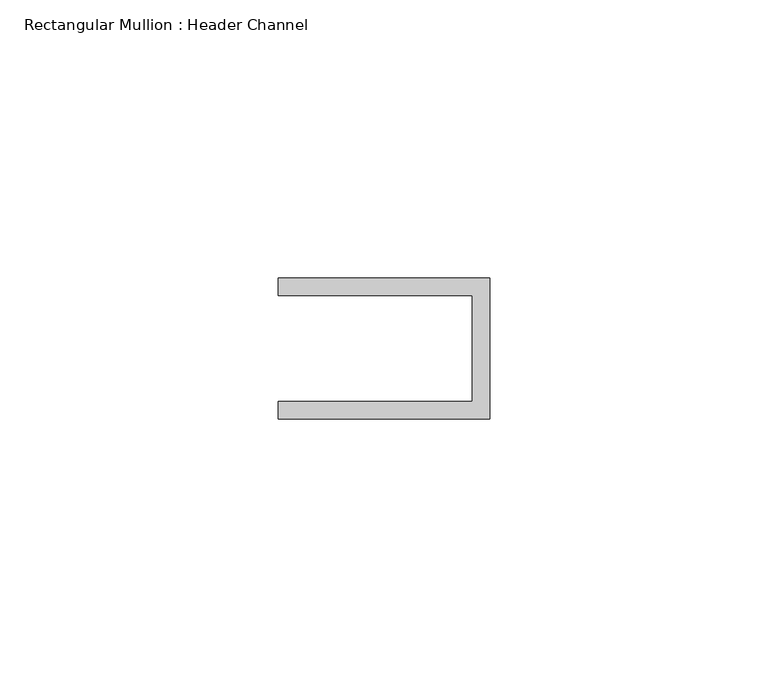
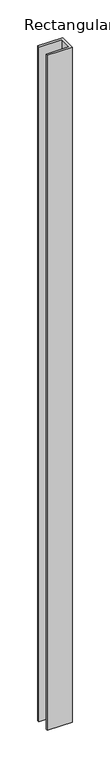
"""IFC4 building model written with IfcOpenShell, lengths in millimetres: member geometry, Rectangular Mullion : Header Channel."""

from ifc_helpers import new_model, si_unit, frame, origin, place, context, project, spatial, polyline, outline, extrude, source, transform, mapped, element, save


def rectangular_mullion_header_channel_626751b6(model_context):
    return source(origin(), model_context, "Body", "SweptSolid", [
        extrude(outline(polyline([(0.0, -12.7), (-38.1, -12.7), (-38.1, -9.525), (-3.175, -9.525), (-3.175, 9.525), (-38.1, 9.525), (-38.1, 12.7), (0.0, 12.7), (0.0, -12.7)])), frame((0.0, 0.0, -1092.2), z_axis=(0.0, 0.0, 1.0), x_axis=(1.0, 0.0, 0.0)), (0.0, 0.0, 1.0), 1092.2),
    ])


if __name__ == "__main__":
    model = new_model("IFC4")
    model_context = context("Model", 3, world=origin())
    ifc_project = project(units=[si_unit("LENGTHUNIT", "METRE", prefix="MILLI")], contexts=[model_context])
    site = spatial("IfcSite", under=ifc_project)
    building = spatial("IfcBuilding", under=site)
    placement = place(None, origin())
    rectangular_mullion_header_channel_shape = rectangular_mullion_header_channel_626751b6(model_context)
    element("IfcMember", 1, ObjectType="Rectangular Mullion : Header Channel", at=placement, inside=building, context=model_context, shape_type="MappedRepresentation", body=[
        mapped(rectangular_mullion_header_channel_shape, transform((0.0, 0.0, 0.0), x_axis=(1.0, 0.0, 0.0), y_axis=(0.0, 1.0, 0.0), z_axis=(0.0, 0.0, 1.0))),
    ])
    save(model, "model.ifc")

# Revit data of these elements
# Type "Rectangular Mullion : Header Channel"
#   built-in parameter 1007322 = 0.0833333 (stored number, unit not read)
#   built-in parameter 1007321 = -0.03125 (stored number, unit not read)
#   built-in parameter 1007320 = 0.0416667 (stored number, unit not read)
# Element 1 (IfcMember, "Rectangular Mullion : Header Channel")
#   Materials on its faces: "ALUM"
# Materials
#   "ALUM": class "Generic", colour RGB 157 157 157, transparency 0, Cost = 0
